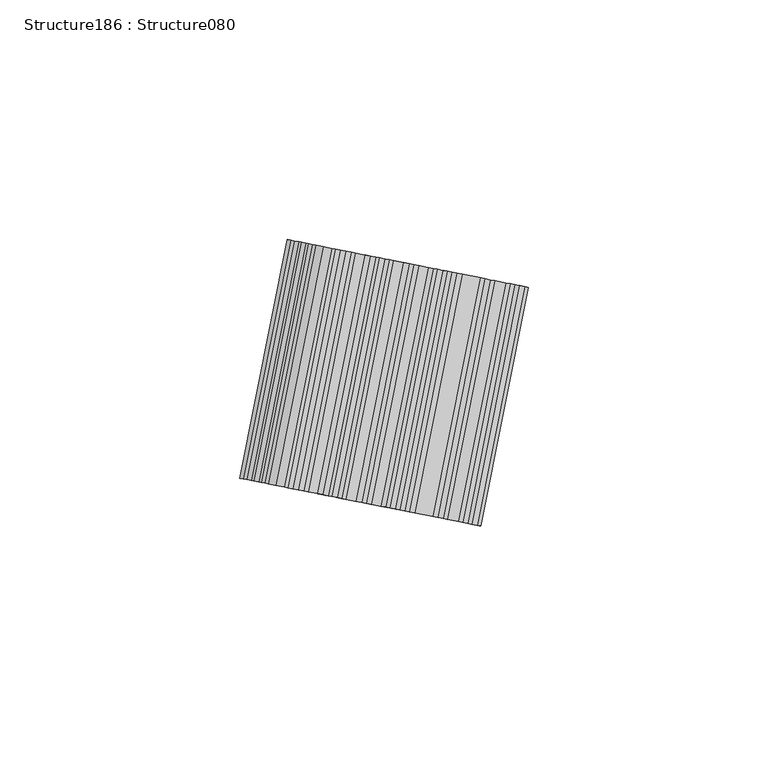
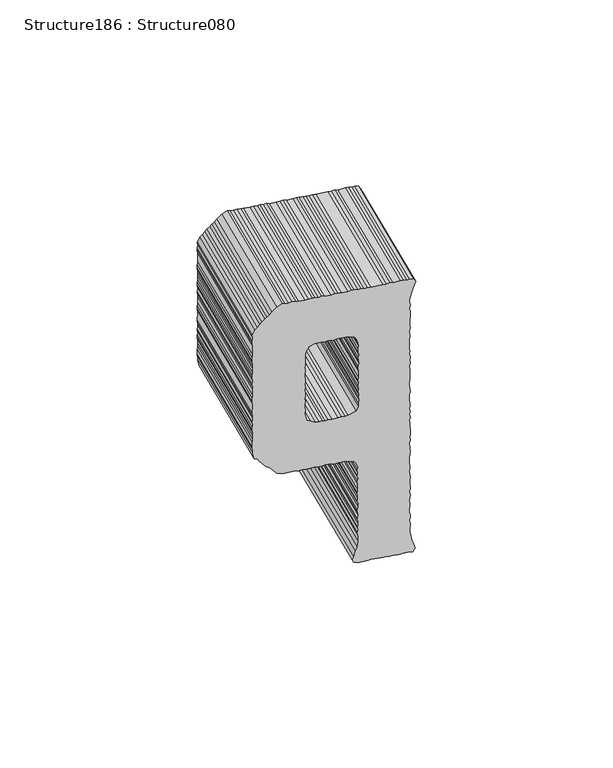
"""IFC4 building model written with IfcOpenShell, lengths in millimetres: proxy geometry, Structure186 : Structure080."""

from ifc_helpers import new_model, si_unit, frame, origin, place, context, project, spatial, polyline, outline, extrude, source, transform, mapped, element, save


def structure186_structure080_8ce57049(model_context):
    return source(origin(), model_context, "Body", "SweptSolid", [
        extrude(outline(polyline([(1.9495147, 0.0), (3.1176578, 0.256899), (4.0285462, 0.1273821), (5.3297645, 0.0), (7.407017, 0.0), (8.3161263, 0.256899), (9.2252356, 0.0), (10.396937, 0.256899), (11.1751061, 0.1273821), (12.3428935, 0.1273821), (13.5145948, 0.0), (15.4644653, 0.1273821), (16.3700164, 0.1273821), (17.5417177, 0.256899), (18.7112842, 0.1273821), (19.7499104, 0.1273821), (20.5280795, 0.256899), (22.3484331, -0.5248282), (23.9061945, -1.9537844), (24.6861427, -2.8628937), (25.4660909, -3.5097668), (25.987361, -4.1623329), (27.0256314, -4.9380113), (27.5451225, -5.7240084), (28.4542317, -6.6270688), (29.2345357, -7.2796349), (30.0141281, -8.9708273), (29.7533152, -10.1368356), (30.0141281, -11.3028439), (30.0141281, -12.0884851), (29.7533152, -13.2541376), (29.7533152, -16.2447692), (30.0141281, -17.2833954), (30.0141281, -18.5824788), (29.7533152, -19.4972812), (29.8846111, -20.4006974), (29.7533152, -21.4396795), (29.8846111, -22.7441001), (30.0141281, -23.6535653), (30.0141281, -24.6864985), (29.8846111, -25.7286829), (30.0141281, -27.0277663), (29.8846111, -28.0667483), (29.7533152, -28.9797716), (29.7533152, -31.0609381), (30.0141281, -32.0931596), (30.0141281, -33.264861), (29.7533152, -34.307757), (30.0141281, -37.425059), (29.8846111, -38.5932022), (29.7533152, -39.3731504), (30.0141281, -40.6722338), (29.8846111, -41.5777849), (30.0141281, -42.6199693), (30.0141281, -43.6585956), (29.8846111, -44.5680607), (29.7533152, -45.7376272), (29.8846111, -46.9096843), (30.0141281, -47.9479548), (30.0141281, -49.7665292), (29.7533152, -50.8090694), (29.7533152, -51.8455608), (29.365476, -53.9228132), (28.3250706, -54.4458624), (27.8055796, -55.2218966), (26.2478181, -57.0401153), (25.595252, -57.6926814), (24.5587606, -58.2121724), (23.2575423, -59.7681548), (22.3484331, -60.8103392), (20.5280795, -61.4589914), (19.7499104, -61.3298302), (18.582123, -61.1963993), (16.3700164, -61.1963993), (15.3331693, -61.4589914), (14.292764, -61.3298302), (13.2523586, -61.4589914), (12.4741894, -61.3298302), (11.1751061, -61.3298302), (10.2659968, -61.1963993), (9.0960745, -61.4589914), (8.3161263, -61.3298302), (7.018822, -61.1963993), (5.0671725, -61.1963993), (3.8972502, -61.4589914), (2.98992, -61.3298302), (2.0808107, -61.3298302), (1.0404054, -61.1963993), (-0.2590338, -61.4589914), (-1.9498704, -61.9763475), (-2.4672265, -62.6289136), (-3.2471747, -64.320106), (-2.9863618, -65.2292153), (-3.1176577, -66.5243847), (-2.9863618, -67.566925), (-3.2471747, -68.4760343), (-2.9863618, -69.3854994), (-3.1176577, -70.6845828), (-3.1176577, -72.6362323), (-2.9863618, -73.6748586), (-3.1176577, -74.7134848), (-3.1176577, -75.7499762), (-2.9863618, -76.9216775), (-3.2471747, -77.7016257), (-3.2471747, -78.8694131), (-2.9863618, -79.9062602), (-3.1176577, -81.0818755), (-3.2471747, -81.9870709), (-2.9863618, -83.1587722), (-3.2471747, -83.9387204), (-3.2471747, -84.9773466), (-3.1176577, -86.270737), (-3.2471747, -87.0563782), (-2.9863618, -88.0950045), (-3.2471747, -89.3940879), (-3.2471747, -91.3421792), (-2.9863618, -93.4229899), (-2.3380654, -94.7163802), (-1.9498704, -96.7975467), (-1.4286003, -97.579274), (-1.9498704, -98.6157653), (-2.9863618, -98.8783574), (-5.1966893, -98.8783574), (-6.3648326, -98.7491962), (-7.2739419, -98.6157653), (-10.3915997, -98.8783574), (-11.3028439, -98.8783574), (-12.3414702, -98.7491962), (-13.2523585, -98.8783574), (-14.2909847, -98.7491962), (-15.4591279, -98.8783574), (-16.4995333, -98.8783574), (-17.2794814, -98.7491962), (-19.4876741, -98.7491962), (-20.3971393, -98.8783574), (-21.1749526, -97.579274), (-20.9184094, -96.7975467), (-20.5263004, -95.7606995), (-20.0089442, -94.4594812), (-19.8776482, -93.6798889), (-19.4876741, -91.3421792), (-19.4876741, -90.4327141), (-19.617191, -89.2667058), (-19.617191, -88.3519035), (-19.358513, -87.3150563), (-19.617191, -86.1472689), (-19.617191, -85.2342456), (-19.358513, -84.3286945), (-19.358513, -83.2865101), (-19.4876741, -81.9870709), (-19.4876741, -81.0818755), (-19.358513, -80.0393353), (-19.4876741, -79.130226), (-19.617191, -78.0876858), (-19.358513, -76.7886024), (-19.617191, -75.8830513), (-19.617191, -74.970028), (-19.4876741, -73.9314017), (-19.4876741, -72.6362323), (-19.617191, -71.723209), (-19.4876741, -70.5572007), (-19.358513, -69.5185745), (-19.4876741, -68.7386263), (-19.4876741, -67.7000001), (-19.358513, -66.3952236), (-19.358513, -64.4474881), (-19.4876741, -63.5380229), (-19.617191, -62.3684565), (-19.4876741, -61.1963993), (-19.358513, -59.1212817), (-19.617191, -58.2121724), (-19.4876741, -57.0401153), (-19.617191, -56.136699), (-19.617191, -54.0558883), (-19.4876741, -53.1407302), (-19.4876741, -51.9747219), (-19.358513, -50.9364514), (-19.617191, -49.8939112), (-19.358513, -48.8570641), (-19.617191, -47.9479548), (-19.358513, -46.6470923), (-19.617191, -45.6102451), (-19.4876741, -44.8285179), (-19.358513, -43.5294345), (-19.358513, -41.5777849), (-19.617191, -40.6722338), (-19.4876741, -39.3731504), (-19.358513, -38.3302544), (-19.358513, -37.2919839), (-19.4876741, -36.2551368), (-19.4876741, -32.2265905), (-19.358513, -31.3135673), (-19.617191, -30.1457799), (-19.4876741, -29.2363148), (-19.617191, -27.9372314), (-19.358513, -26.90074), (-19.4876741, -25.9916307), (-19.358513, -25.0803865), (-19.358513, -21.7001367), (-19.4876741, -20.6632895), (-19.4876741, -19.8812064), (-19.358513, -18.71164), (-19.617191, -17.5438526), (-19.4876741, -16.6343875), (-19.4876741, -14.4258389), (-19.617191, -13.5170855), (-19.617191, -11.4362748), (-19.358513, -10.5268097), (-19.617191, -9.2334193), (-19.358513, -7.4091519), (-19.8776482, -5.0714422), (-20.2658432, -4.032816), (-20.5263004, -2.9959688), (-20.9184094, -2.2142415), (-21.3062485, -1.0443193), (-20.5263004, 0.1273821), (-19.358513, 0.256899), (-18.4490479, 0.0), (-17.4086425, 0.256899), (-16.4995333, 0.256899), (-14.1618236, 0.0), (-13.2523585, 0.256899), (-12.0806572, 0.0), (-11.0441658, 0.1273821), (-7.2739419, 0.0), (-6.1061545, 0.1273821), (-5.0675282, 0.0), (-4.0271229, 0.1273821), (-3.1176577, 0.0), (-1.9498704, 0.256899), (-1.0386262, 0.256899), (0.0, 0.0), (1.9495147, 0.0)]), holes=[polyline([(-2.5985226, -43.6585956), (0.0, -44.8285179), (0.9108884, -44.9580348), (2.0808107, -44.8285179), (3.1176578, -44.9580348), (5.0671725, -45.085061), (6.2388739, -44.9580348), (7.275721, -45.085061), (8.0556692, -44.9580348), (9.0960745, -45.085061), (10.2659968, -44.9580348), (11.8237582, -44.1816448), (12.7350024, -43.7916707), (13.1228416, -41.9734521), (13.3832988, -41.1917248), (13.1228416, -39.8926414), (13.3832988, -38.8536594), (13.3832988, -37.8168122), (13.2523586, -36.7728487), (13.3832988, -35.7360015), (13.2523586, -34.8211992), (13.1228416, -33.784352), (13.3832988, -32.7460816), (13.1228416, -31.5743802), (13.3832988, -30.7979902), (13.2523586, -29.7558058), (13.2523586, -28.8463407), (13.3832988, -27.8094935), (13.3832988, -26.6377922), (13.1228416, -25.5995217), (13.3832988, -24.4331576), (13.1228416, -23.6535653), (13.2523586, -22.4818639), (13.1228416, -21.3101626), (13.2523586, -20.4006974), (13.1228416, -19.3645619), (12.4741894, -17.9356058), (12.0863503, -17.1538785), (10.396937, -16.5016682), (8.3161263, -16.5016682), (7.018822, -16.6343875), (6.1075778, -16.3739303), (4.9380114, -16.6343875), (4.1580631, -16.5016682), (3.1176578, -16.3739303), (-0.1295169, -16.3739303), (-2.0772524, -17.0264964), (-2.7276837, -17.8060888), (-3.1176577, -19.3645619), (-3.2471747, -20.4006974), (-3.1176577, -21.4396795), (-3.1176577, -22.6152948), (-3.3763359, -23.6535653), (-3.1176577, -24.4331576), (-3.2471747, -25.7286829), (-3.3763359, -26.6377922), (-3.1176577, -27.6806882), (-3.1176577, -28.5897975), (-3.2471747, -29.6223749), (-3.2471747, -31.7031855), (-3.1176577, -32.8791567), (-3.2471747, -33.6555467), (-3.1176577, -34.8211992), (-3.2471747, -35.9989494), (-3.1176577, -36.9023656), (-3.3763359, -38.0680181), (-3.2471747, -38.8536594), (-3.3763359, -39.8926414), (-3.2471747, -41.1917248), (-3.2471747, -42.2299952), (-2.5985226, -43.6585956)])]), frame((-1655.8424977, 234797.0941845, 485.2778019), z_axis=(0.1946622229639412, 0.9808703374813293, 0.0), x_axis=(-0.9808703374813293, 0.1946622229639412, 0.0)), (0.0, 0.0, 1.0), 50.8),
    ])


if __name__ == "__main__":
    model = new_model("IFC4")
    model_context = context("Model", 3, world=origin())
    ifc_project = project(units=[si_unit("LENGTHUNIT", "METRE", prefix="MILLI")], contexts=[model_context])
    site = spatial("IfcSite", under=ifc_project)
    building = spatial("IfcBuilding", under=site)
    placement = place(None, origin())
    structure186_structure080_shape = structure186_structure080_8ce57049(model_context)
    element("IfcBuildingElementProxy", 1, Name="Structure186 : Structure080", ObjectType="Structure186 : Structure080", at=placement, inside=building, context=model_context, shape_type="MappedRepresentation", body=[
        mapped(structure186_structure080_shape, transform((0.0, 0.0, 0.0), x_axis=(1.0, 0.0, 0.0), y_axis=(0.0, 1.0, 0.0), z_axis=(0.0, 0.0, 1.0))),
    ])
    save(model, "model.ifc")

# Revit data of these elements
# Type "Structure186 : Structure080"
#   NameOverride = "Structure080"
# Element 1 (IfcBuildingElementProxy, "Structure186 : Structure080")
#   Materials on its faces: "BRUSHED ALUMINUM LETTERING"
# Materials
#   "BRUSHED ALUMINUM LETTERING": class "Unassigned", colour RGB 169 181 186, transparency 0, Cost = 0
